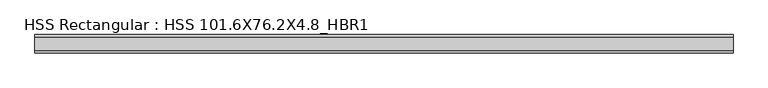
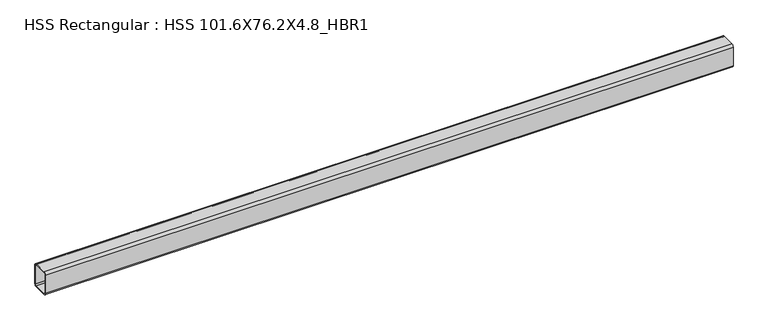
"""IFC4 building model written with IfcOpenShell, lengths in millimetres: beam geometry, HSS Rectangular : HSS 101.6X76.2X4.8_HBR1."""

from ifc_helpers import new_model, si_unit, point, frame, frame_2d, origin, place, context, project, spatial, polyline, circle_curve, trimmed, segment, composite_curve, outline, extrude, source, transform, mapped, element, save


def hss_rectangular_hss_101_6x76_2x4_8_hbr1_c561afbc(model_context):
    return source(origin(), model_context, "Body", "SweptSolid", [
        extrude(outline(composite_curve([segment(polyline([(38.1, 41.275), (38.1, -41.275)]), True, "CONTINUOUS"), segment(trimmed(circle_curve(frame_2d((28.575, -41.275)), 9.525), [point((38.1, -41.275))], [point((28.575, -50.8))], False, "CARTESIAN"), True, "CONTINUOUS"), segment(polyline([(28.575, -50.8), (-28.575, -50.8)]), True, "CONTINUOUS"), segment(trimmed(circle_curve(frame_2d((-28.575, -41.275)), 9.525), [point((-28.575, -50.8))], [point((-38.1, -41.275))], False, "CARTESIAN"), True, "CONTINUOUS"), segment(polyline([(-38.1, -41.275), (-38.1, 41.275)]), True, "CONTINUOUS"), segment(trimmed(circle_curve(frame_2d((-28.575, 41.275)), 9.525), [point((-38.1, 41.275))], [point((-28.575, 50.8))], False, "CARTESIAN"), True, "CONTINUOUS"), segment(polyline([(-28.575, 50.8), (28.575, 50.8)]), True, "CONTINUOUS"), segment(trimmed(circle_curve(frame_2d((28.575, 41.275)), 9.525), [point((28.575, 50.8))], [point((38.1, 41.275))], False, "CARTESIAN"), True, "CONTINUOUS")], self_intersect=False), holes=[composite_curve([segment(trimmed(circle_curve(frame_2d((-28.575, 41.275)), 4.7625), [point((-28.575, 46.0375))], [point((-33.3375, 41.275))], True, "CARTESIAN"), True, "CONTINUOUS"), segment(polyline([(-33.3375, 41.275), (-33.3375, -41.275)]), True, "CONTINUOUS"), segment(trimmed(circle_curve(frame_2d((-28.575, -41.275)), 4.7625), [point((-33.3375, -41.275))], [point((-28.575, -46.0375))], True, "CARTESIAN"), True, "CONTINUOUS"), segment(polyline([(-28.575, -46.0375), (28.575, -46.0375)]), True, "CONTINUOUS"), segment(trimmed(circle_curve(frame_2d((28.575, -41.275)), 4.7625), [point((28.575, -46.0375))], [point((33.3375, -41.275))], True, "CARTESIAN"), True, "CONTINUOUS"), segment(polyline([(33.3375, -41.275), (33.3375, 41.275)]), True, "CONTINUOUS"), segment(trimmed(circle_curve(frame_2d((28.575, 41.275)), 4.7625), [point((33.3375, 41.275))], [point((28.575, 46.0375))], True, "CARTESIAN"), True, "CONTINUOUS"), segment(polyline([(28.575, 46.0375), (-28.575, 46.0375)]), True, "CONTINUOUS")], self_intersect=False)]), frame((-1460.0, 0.0, 0.0), z_axis=(1.0, 0.0, 0.0), x_axis=(0.0, 1.0, 0.0)), (0.0, 0.0, 1.0), 2920.0),
    ])


if __name__ == "__main__":
    model = new_model("IFC4")
    model_context = context("Model", 3, world=origin())
    ifc_project = project(units=[si_unit("LENGTHUNIT", "METRE", prefix="MILLI")], contexts=[model_context])
    site = spatial("IfcSite", under=ifc_project)
    building = spatial("IfcBuilding", under=site)
    placement = place(None, origin())
    hss_rectangular_hss_101_6x76_2x4_8_hbr1_shape = hss_rectangular_hss_101_6x76_2x4_8_hbr1_c561afbc(model_context)
    element("IfcBeam", 1, ObjectType="HSS Rectangular : HSS 101.6X76.2X4.8_HBR1", at=placement, inside=building, context=model_context, shape_type="MappedRepresentation", body=[
        mapped(hss_rectangular_hss_101_6x76_2x4_8_hbr1_shape, transform((0.0, 0.0, 0.0), x_axis=(1.0, 0.0, 0.0), y_axis=(0.0, 1.0, 0.0), z_axis=(0.0, 0.0, 1.0))),
    ])
    save(model, "model.ifc")

# Revit data of these elements
# Type "HSS Rectangular : HSS 101.6X76.2X4.8_HBR1"
#   Section Name Key = "HSS 4X3X3/16"
#   Assembly Code = "B10"
#   Width = 7.62 cm
#   Wall Nominal Thickness = 0.4763 cm
#   Wall Design Thickness = 0.442 cm
#   Torsional Moment of Inertia = 260.561 cm⁴
#   Torsional Modulus = 61.2876 cm³
#   Section Area = 14.4516 cm²
#   Plastic Modulus weak axis = 40.3122 cm³
#   Plastic Modulus strong axis = 49.1612 cm³
#   Perimeter = 0.881482 m²/m
#   Outer Fillet = 0.9525 cm
#   Nominal Weight = 12.1285 kgf/m
#   Moment of Inertia weak axis = 131.529 cm⁴
#   Moment of Inertia strong axis = 205.202 cm⁴
#   Inner Fillet = 0.4763 cm
#   Height = 10.16 cm
#   Elastic Modulus weak axis = 34.4128 cm³
#   Elastic Modulus strong axis = 40.476 cm³
#   Centroid Vertical = 5.08 cm
#   Centroid Horizontal = 3.81 cm
#   Length [instance default] = 1524 mm
#   Structural Material [instance default] = Steel ASTM A500, Grade B, Rectangular and Square
#   Principal Axes Angle = 0
# Element 1 (IfcBeam, "HSS Rectangular : HSS 101.6X76.2X4.8_HBR1")
#   Structural Material = Steel ASTM A992
#   Materials on its faces: "Steel ASTM A992"
# Materials
#   "Steel ASTM A500, Grade B, Rectangular and Square": class "Metal", colour RGB 199 199 199, transparency 0, Description = "Carbon steel", Cost = 0
#   "Steel ASTM A992": class "Metal", colour RGB 199 199 199, transparency 0, Description = "Structural steel 50ksi", Cost = 0
